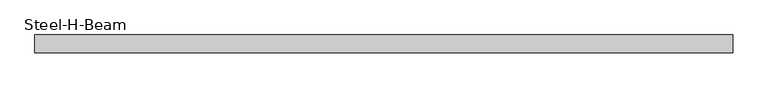
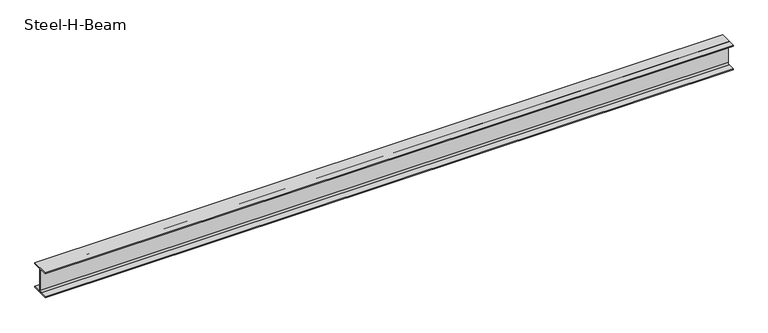
"""IFC4 building model written with IfcOpenShell, lengths in millimetres: beam geometry, Steel-H-Beam : BM121_H-294×200x8x12."""

from ifc_helpers import new_model, si_unit, point, frame, frame_2d, origin, place, context, project, spatial, polyline, circle_curve, trimmed, segment, composite_curve, outline, extrude, source, transform, mapped, element, save


def steel_h_beam_f2b553ac(model_context):
    return source(origin(), model_context, "Body", "SweptSolid", [
        extrude(outline(composite_curve([segment(polyline([(100.0, -135.0), (100.0, -147.0), (-100.0, -147.0), (-100.0, -135.0), (-22.0, -135.0)]), True, "CONTINUOUS"), segment(trimmed(circle_curve(frame_2d((-22.0, -117.0)), 18.0), [point((-22.0, -135.0))], [point((-4.0, -117.0))], True, "CARTESIAN"), True, "CONTINUOUS"), segment(polyline([(-4.0, -117.0), (-4.0, 117.0)]), True, "CONTINUOUS"), segment(trimmed(circle_curve(frame_2d((-22.0, 117.0)), 18.0), [point((-4.0, 117.0))], [point((-22.0, 135.0))], True, "CARTESIAN"), True, "CONTINUOUS"), segment(polyline([(-22.0, 135.0), (-100.0, 135.0), (-100.0, 147.0), (100.0, 147.0), (100.0, 135.0), (22.0, 135.0)]), True, "CONTINUOUS"), segment(trimmed(circle_curve(frame_2d((22.0, 117.0)), 18.0), [point((22.0, 135.0))], [point((4.0, 117.0))], True, "CARTESIAN"), True, "CONTINUOUS"), segment(polyline([(4.0, 117.0), (4.0, -117.0)]), True, "CONTINUOUS"), segment(trimmed(circle_curve(frame_2d((22.0, -117.0)), 18.0), [point((4.0, -117.0))], [point((22.0, -135.0))], True, "CARTESIAN"), True, "CONTINUOUS"), segment(polyline([(22.0, -135.0), (100.0, -135.0)]), True, "CONTINUOUS")], self_intersect=False)), frame((-3861.3486745, 0.0, 0.0), z_axis=(1.0, 0.0, 0.0), x_axis=(0.0, 1.0, 0.0)), (0.0, 0.0, 1.0), 7724.6),
    ])


if __name__ == "__main__":
    model = new_model("IFC4")
    model_context = context("Model", 3, world=origin())
    ifc_project = project(units=[si_unit("LENGTHUNIT", "METRE", prefix="MILLI")], contexts=[model_context])
    site = spatial("IfcSite", under=ifc_project)
    building = spatial("IfcBuilding", under=site)
    placement = place(None, origin())
    steel_h_beam_shape = steel_h_beam_f2b553ac(model_context)
    element("IfcBeam", 1, ObjectType="Steel-H-Beam : BM121_H-294×200x8x12", at=placement, inside=building, context=model_context, shape_type="MappedRepresentation", body=[
        mapped(steel_h_beam_shape, transform((0.0, 0.0, 0.0), x_axis=(1.0, 0.0, 0.0), y_axis=(0.0, 1.0, 0.0), z_axis=(0.0, 0.0, 1.0))),
    ])
    save(model, "model.ifc")

# Revit data of these elements
# Type "Steel-H-Beam : BM121_H-294×200x8x12"
#   Surface Area = 1.3411 m²/m
#   Section Area = 72.3812 cm²
#   Mass per Unit Length = 56.8193 kg/m
#   Length [instance default] = 3000 mm
#   B = 200 mm
#   H = 294 mm
#   r = 18 mm
#   tw = 8 mm
#   tf = 12 mm
#   hec_material4 [instance default] = none
#   hec_material3 [instance default] = none
#   hec_material2 [instance default] = none
#   hec_material1 [instance default] = none
#   Structural Material [instance default] = Steel, 45-345
#   Assembly Code = ""
# Element 1 (IfcBeam, "Steel-H-Beam : BM121_H-294×200x8x12")
#   hec_material3 = F01AC000-00002_Building/Shelter Fire Proofing Work_Intumescent Coating Type_1 hr. rating (UL 1709))
#   hec_material2 = S01AA010-00002_Main Steel Structure Fabrication Work_Shelter/Building_Steel Painting/Coating_for Fireproofed Steel Surface, Surface Preparation & Primer Coat
#   hec_material1 = S03AA028-00001_Main Steel Structure Erection Work_Shelter/Building_Medium Steel
#   Structural Material = S01AA002-00001_Main Steel Structure Fabrication Work_Shelter/Building_Medium Steel - Standard
#   Materials on its faces: "S01AA002-00001_Main Steel Structure Fabrication Work_Shelter/Building_Medium Steel - Standard"
# Materials
#   "Steel, 45-345": class "Metal", colour RGB 189 187 185, transparency 0, Description = "Steel 345 MPa", Cost = 0
#   "S01AA002-00001_Main Steel Structure Fabrication Work_Shelter/Building_Medium Steel - Standard": class "Metal", colour RGB 120 120 120, transparency 0, Comments = "(90KG/M>Weight≥30KG/M)", Description = "Structural steel 50ksi", W00) Work Master Code = "S01AA002-0001", W01) Work Master_Lv1 = "Main Steel Structure Fabrication Work", W02) Work Master_Lv2 = "Shelter/Building", W03) Work Master_Spec.1 = "Medium Steel - Standard (90KG/M>Weight≥30KG/M)", Cost = 0
#   "F01AC000-00002_Building/Shelter Fire Proofing Work_Intumescent Coating Type_1 hr. rating (UL 1709))": class "Metal", colour RGB 255 128 128, transparency 0, Description = "Paint finished steel", W00) Work Master Code = "F01AC000-00002", W01) Work Master_Lv1 = "Building/Shelter Fire Proofing Work", W02) Work Master_Lv2 = "Intumescent Coating Type", W03) Work Master_Spec.1 = "1 hr. rating (UL 1709)", Cost = 0
#   "S01AA010-00002_Main Steel Structure Fabrication Work_Shelter/Building_Steel Painting/Coating_for Fireproofed Steel Surface, Surface Preparation & Primer Coat": class "Metal", colour RGB 120 120 120, transparency 0, Description = "Paint finished steel", W00) Work Master Code = "SS01AA010-00002", W01) Work Master_Lv1 = "Main Steel Structure Fabrication Work", W02) Work Master_Lv2 = "Shelter/Building", W03) Work Master_Spec.1 = "Steel Painting/Coating", W04) Work Master_Spec.2 = "for Fireproofed Steel Surface, Surface Preparation & Primer Coat", Cost = 0
#   "S03AA028-00001_Main Steel Structure Erection Work_Shelter/Building_Medium Steel": class "Metal", colour RGB 120 120 120, transparency 0, Comments = "(90KG/M>Weight≥30KG/M)", Description = "Structural steel 50ksi", W00) Work Master Code = "S03AA028-0001", W01) Work Master_Lv1 = "Main Steel Structure Erection Work", W02) Work Master_Lv2 = "Shelter/Building", W03) Work Master_Spec.1 = "Medium Steel (90KG/M>Weight≥30KG/M)", Cost = 0
